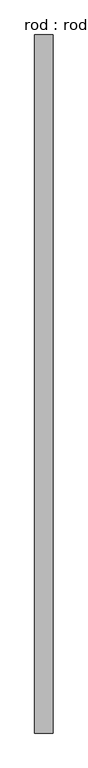
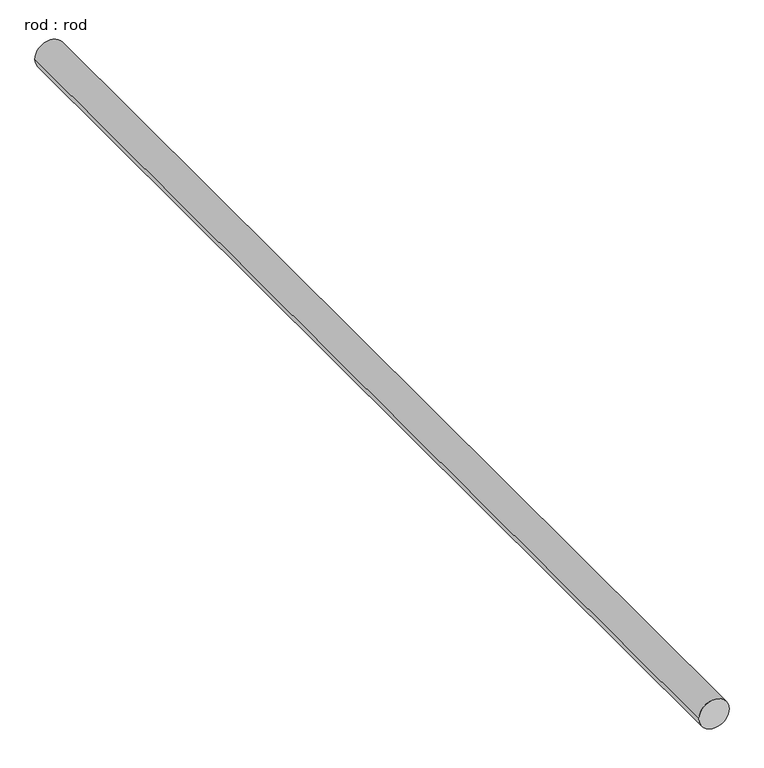
"""IFC4 building model written with IfcOpenShell, lengths in millimetres: proxy geometry, rod : rod."""

from ifc_helpers import new_model, si_unit, point, frame, frame_2d, origin, place, context, project, spatial, circle_curve, trimmed, segment, composite_curve, outline, extrude, source, transform, mapped, element, save


def rod_rod_5f88a9b5(model_context):
    return source(origin(), model_context, "Body", "SweptSolid", [
        extrude(outline(composite_curve([segment(trimmed(circle_curve(frame_2d((0.0108462, 0.0)), 200.0), [point((0.0108462, 200.0))], [point((0.0108462, -200.0))], False, "CARTESIAN"), True, "CONTINUOUS"), segment(trimmed(circle_curve(frame_2d((0.0108462, 0.0)), 200.0), [point((0.0108462, -200.0))], [point((0.0108462, 200.0))], False, "CARTESIAN"), True, "CONTINUOUS")], self_intersect=False)), frame((0.0, -3527.8070989, 0.0), z_axis=(0.0, 1.0, 0.0), x_axis=(0.0, 0.0, 1.0)), (0.0, 0.0, 1.0), 15241.0714286),
    ])


if __name__ == "__main__":
    model = new_model("IFC4")
    model_context = context("Model", 3, world=origin())
    ifc_project = project(units=[si_unit("LENGTHUNIT", "METRE", prefix="MILLI")], contexts=[model_context])
    site = spatial("IfcSite", under=ifc_project)
    building = spatial("IfcBuilding", under=site)
    placement = place(None, origin())
    rod_rod_shape = rod_rod_5f88a9b5(model_context)
    element("IfcBuildingElementProxy", 1, Name="rod : rod", ObjectType="rod : rod", at=placement, inside=building, context=model_context, shape_type="MappedRepresentation", body=[
        mapped(rod_rod_shape, transform((0.0, 0.0, 0.0), x_axis=(1.0, 0.0, 0.0), y_axis=(0.0, 1.0, 0.0), z_axis=(0.0, 0.0, 1.0))),
    ])
    save(model, "model.ifc")

# Revit data of these elements
# Type "rod : rod"
#   Default Elevation = 0
